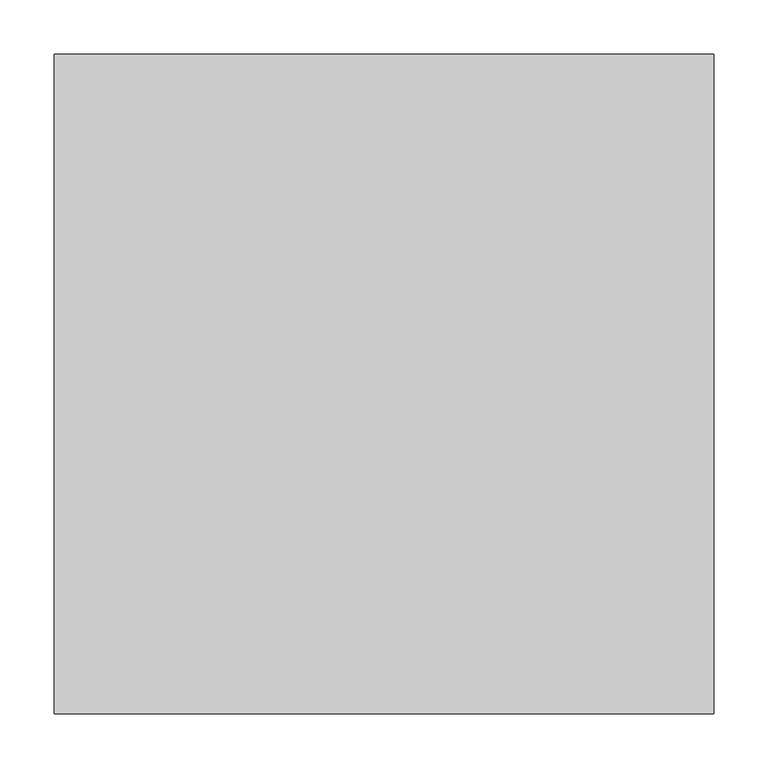
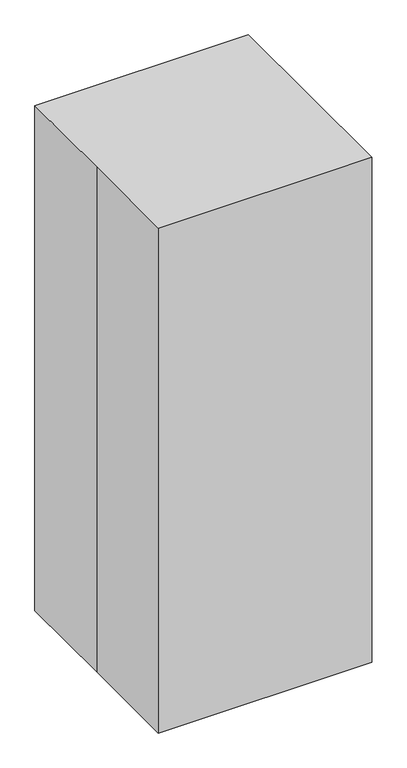
"""IFC4 building model written with IfcOpenShell, lengths in millimetres: proxy geometry, M4116 - Monitor, Vital Signs, On Mobile Stand : M4116 - Monitor, Vital Signs, On Mobile Stand."""

import ifcopenshell
import ifcopenshell.guid

model = None  # the IFC model being written
_history = None  # IfcOwnerHistory: only IFC2X3 demands one
_inside = {}  # id of a spatial element -> (the spatial element, [elements in it])
_under = {}  # id of a project, library or spatial element -> (it, [spatial elements below it])
_declared = {}  # id of a project -> (the project, [libraries it declares])
_typed = {}  # id of a type object -> (the type object, [elements of that type])
_made_of = {}  # id of a material, layer set ... -> (it, [elements and type objects made of it])


def new_model(schema):
    """Start an empty IFC model of exactly this schema.

    Asked for "IFC4X3", IfcOpenShell would pick the latest addendum, in which some entities
    have other attributes; the version numbers below select the first issue.
    IFC2X3 requires an IfcOwnerHistory on every rooted entity: one is made here for all.
    """
    global model, _history
    if schema == "IFC4X3":
        model = ifcopenshell.file(schema_version=(4, 3, 0, 0))
    else:
        model = ifcopenshell.file(schema=schema)
    _inside.clear()
    _under.clear()
    _declared.clear()
    _typed.clear()
    _made_of.clear()
    _history = None
    if model.schema == "IFC2X3":
        org = make("IfcOrganization", Name="unknown")
        user = make(
            "IfcPersonAndOrganization",
            ThePerson=make("IfcPerson", FamilyName="unknown"),
            TheOrganization=org,
        )
        app = make(
            "IfcApplication",
            ApplicationDeveloper=org,
            Version="unknown",
            ApplicationFullName="unknown",
            ApplicationIdentifier="unknown",
        )
        _history = make(
            "IfcOwnerHistory",
            OwningUser=user,
            OwningApplication=app,
            ChangeAction="ADDED",
            CreationDate=0,
        )
    return model


def make(cls, **values):
    """One entity of the class cls with the attributes given. An attribute that is None is left unset."""
    return model.create_entity(
        cls, **{name: value for name, value in values.items() if value is not None}
    )


def rooted(cls, **values):
    """An entity with a GlobalId (a new one), such as an element, a storey or a relation."""
    return make(cls, GlobalId=ifcopenshell.guid.new(), OwnerHistory=_history, **values)


def si_unit(unit_type, name, prefix=None):
    """IfcSIUnit, for example si_unit("LENGTHUNIT", "METRE", prefix="MILLI")."""
    return make("IfcSIUnit", UnitType=unit_type, Prefix=prefix, Name=name)


def assignment(units):
    """IfcUnitAssignment: the units of a project."""
    return None if units is None else make("IfcUnitAssignment", Units=units)


def point(xyz):
    """IfcCartesianPoint."""
    return None if xyz is None else make("IfcCartesianPoint", Coordinates=xyz)


def direction(xyz):
    """IfcDirection."""
    return None if xyz is None else make("IfcDirection", DirectionRatios=xyz)


def frame(location, z_axis=None, x_axis=None):
    """IfcAxis2Placement3D, a coordinate frame: its origin and axes. An axis left out is left unset."""
    return make(
        "IfcAxis2Placement3D",
        Location=point(location),
        Axis=direction(z_axis),
        RefDirection=direction(x_axis),
    )


def frame_2d(location, x_axis=None):
    """IfcAxis2Placement2D, a coordinate frame in the plane: its origin and x axis."""
    return make(
        "IfcAxis2Placement2D", Location=point(location), RefDirection=direction(x_axis)
    )


def origin():
    """The frame at (0, 0, 0) with its axes left unset."""
    return frame((0.0, 0.0, 0.0))


def origin_with_axes():
    """The frame at (0, 0, 0) with the z axis (0, 0, 1) and the x axis (1, 0, 0) written out."""
    return frame((0.0, 0.0, 0.0), z_axis=(0.0, 0.0, 1.0), x_axis=(1.0, 0.0, 0.0))


def origin_2d():
    """The frame at (0, 0) in the plane with its x axis left unset."""
    return frame_2d((0.0, 0.0))


def place(relative_to, where):
    """IfcLocalPlacement: puts the frame where relative to a parent placement (None: the world)."""
    return make(
        "IfcLocalPlacement", PlacementRelTo=relative_to, RelativePlacement=where
    )


def context(
    kind, dimensions, precision=None, world=None, true_north=None, identifier=None
):
    """IfcGeometricRepresentationContext, for example the 3D "Model" context."""
    return make(
        "IfcGeometricRepresentationContext",
        ContextIdentifier=identifier,
        ContextType=kind,
        CoordinateSpaceDimension=dimensions,
        Precision=precision,
        WorldCoordinateSystem=world,
        TrueNorth=true_north,
    )


def project(units=None, contexts=None):
    """IfcProject with its units and contexts."""
    return rooted(
        "IfcProject",
        Name="project",
        RepresentationContexts=contexts,
        UnitsInContext=assignment(units),
    )


def spatial(cls, under=None, at=None, **own):
    """A site, building, storey or space (cls), placed at a placement, below another one or the project."""
    s = rooted(cls, ObjectPlacement=at, **own)
    if under is not None:
        _under.setdefault(under.id(), (under, []))[1].append(s)
    return s


def polyline(points):
    """IfcPolyline through the points."""
    return make("IfcPolyline", Points=[point(p) for p in points])


def circle_curve(where, radius):
    """IfcCircle in the frame where."""
    return make("IfcCircle", Position=where, Radius=radius)


def ellipse_curve(where, semi_axis1, semi_axis2):
    """IfcEllipse in the frame where."""
    return make(
        "IfcEllipse", Position=where, SemiAxis1=semi_axis1, SemiAxis2=semi_axis2
    )


def trimmed(basis, trim1, trim2, sense, master):
    """IfcTrimmedCurve: the piece of a basis curve between two trims."""
    return make(
        "IfcTrimmedCurve",
        BasisCurve=basis,
        Trim1=trim1,
        Trim2=trim2,
        SenseAgreement=sense,
        MasterRepresentation=master,
    )


def segment(curve, same_sense, transition):
    """IfcCompositeCurveSegment."""
    return make(
        "IfcCompositeCurveSegment",
        Transition=transition,
        SameSense=same_sense,
        ParentCurve=curve,
    )


def composite_curve(segments, self_intersect=None):
    """IfcCompositeCurve: segments joined end to end."""
    return make("IfcCompositeCurve", Segments=segments, SelfIntersect=self_intersect)


def outline(outer, holes=None, kind="AREA"):
    """IfcArbitraryClosedProfileDef: a profile drawn as a closed curve; with holes, ...WithVoids."""
    if holes is None:
        return make("IfcArbitraryClosedProfileDef", ProfileType=kind, OuterCurve=outer)
    return make(
        "IfcArbitraryProfileDefWithVoids",
        ProfileType=kind,
        OuterCurve=outer,
        InnerCurves=holes,
    )


def extrude(swept, where, along, depth):
    """IfcExtrudedAreaSolid: the profile swept, set in the frame where, extruded along a direction by depth."""
    return make(
        "IfcExtrudedAreaSolid",
        SweptArea=swept,
        Position=where,
        ExtrudedDirection=direction(along),
        Depth=depth,
    )


def shape(context_of_items, identifier, shape_type, items):
    """IfcShapeRepresentation: the items that make up one representation, for example the "Body"."""
    return make(
        "IfcShapeRepresentation",
        ContextOfItems=context_of_items,
        RepresentationIdentifier=identifier,
        RepresentationType=shape_type,
        Items=items,
    )


def source(mapping_origin, context_of_items, identifier, shape_type, items):
    """IfcRepresentationMap: a shape defined once, which mapped items show again and again."""
    return make(
        "IfcRepresentationMap",
        MappingOrigin=mapping_origin,
        MappedRepresentation=shape(context_of_items, identifier, shape_type, items),
    )


def transform(
    local_origin,
    x_axis=None,
    y_axis=None,
    z_axis=None,
    scale=None,
    scale2=None,
    scale3=None,
    uniform=True,
):
    """IfcCartesianTransformationOperator3D, or its non-uniform kind. x_axis, y_axis, z_axis: its Axis1, 2, 3."""
    if uniform:
        return make(
            "IfcCartesianTransformationOperator3D",
            Axis1=direction(x_axis),
            Axis2=direction(y_axis),
            LocalOrigin=point(local_origin),
            Scale=scale,
            Axis3=direction(z_axis),
        )
    return make(
        "IfcCartesianTransformationOperator3DnonUniform",
        Axis1=direction(x_axis),
        Axis2=direction(y_axis),
        LocalOrigin=point(local_origin),
        Scale=scale,
        Axis3=direction(z_axis),
        Scale2=scale2,
        Scale3=scale3,
    )


def mapped(mapping_source, mapping_target):
    """IfcMappedItem: shows the shape of a source again, moved by a transform."""
    return make(
        "IfcMappedItem", MappingSource=mapping_source, MappingTarget=mapping_target
    )


def made_of(thing, what):
    """Note that an element or type object is made of a material, layer set ...; save() writes the relation."""
    if what is not None:
        _made_of.setdefault(what.id(), (what, []))[1].append(thing)
    return thing


def element(
    cls,
    number,
    at=None,
    inside=None,
    cuts=None,
    type_object=None,
    material=None,
    context=None,
    identifier="Body",
    shape_type=None,
    held_by="IfcProductDefinitionShape",
    body=None,
    shapes=None,
    **own,
):
    """One element of the class cls, such as IfcWall. Its Tag is "e" and its number.

    at: its placement. inside: the storey or other place that contains it. cuts: it is an
    opening in that element (IfcRelVoidsElement). A single representation is given by context,
    identifier, shape_type and body (its items); several are given by shapes. held_by: the class
    of the entity that holds the representations. save() writes the other relations.
    """
    e = rooted(cls, Tag="e%d" % number, ObjectPlacement=at, **own)
    if body is not None:
        shapes = [shape(context, identifier, shape_type, body)]
    if shapes is not None:
        e.Representation = make(held_by, Representations=shapes)
    if inside is not None:
        _inside.setdefault(inside.id(), (inside, []))[1].append(e)
    if cuts is not None:
        rooted(
            "IfcRelVoidsElement", RelatingBuildingElement=cuts, RelatedOpeningElement=e
        )
    if type_object is not None:
        _typed.setdefault(type_object.id(), (type_object, []))[1].append(e)
    return made_of(e, material)


def aggregate(whole, parts):
    """IfcRelAggregates: a whole, such as a stair, and the parts it consists of."""
    return rooted("IfcRelAggregates", RelatingObject=whole, RelatedObjects=parts)


def save(model, path):
    """Write the relations noted so far, then the file.

    IfcRelAggregates (storeys below a building ...), IfcRelContainedInSpatialStructure (elements
    in a storey), IfcRelDefinesByType, IfcRelAssociatesMaterial and IfcRelDeclares: one each for
    every whole, place, type object, material and project.
    """
    for whole, parts in _under.values():
        aggregate(whole, parts)
    for where, things in _inside.values():
        rooted(
            "IfcRelContainedInSpatialStructure",
            RelatedElements=things,
            RelatingStructure=where,
        )
    for kind, things in _typed.values():
        rooted("IfcRelDefinesByType", RelatedObjects=things, RelatingType=kind)
    for what, things in _made_of.values():
        rooted("IfcRelAssociatesMaterial", RelatedObjects=things, RelatingMaterial=what)
    for by, libraries in _declared.values():
        rooted("IfcRelDeclares", RelatingContext=by, RelatedDefinitions=libraries)
    model.write(path)


def plane_surface(at):
    """IfcPlane: the flat surface through the origin of the frame at, square to its z axis."""
    return make("IfcPlane", Position=at)


def cylinder_surface(at, radius):
    """IfcCylindricalSurface: all points at the distance radius from the z axis of the frame at."""
    return make("IfcCylindricalSurface", Position=at, Radius=radius)


def advanced_brep(points, edges, surfaces, faces):
    """IfcAdvancedBrep: a solid bounded by faces that lie on surfaces and meet in shared edges.

    An edge is (start, end): straight between two places in points (the first is 0);
    or (start, end, curve); or (start, end, curve, False) where it runs against its curve.
    A face is (place in surfaces, loops), or (place, loops, False) where it looks against
    its surface's normal. A loop lists edges by number (the first is 1), with a minus sign
    where the edge is run from its end to its start. The first loop is the outer one.
    """
    corners = [point(p) for p in points]
    vertices = [make("IfcVertexPoint", VertexGeometry=c) for c in corners]
    made = []
    for start, end, *more in edges:
        made.append(
            make(
                "IfcEdgeCurve",
                EdgeStart=vertices[start],
                EdgeEnd=vertices[end],
                EdgeGeometry=more[0] if more else make("IfcPolyline", Points=[corners[start], corners[end]]),
                SameSense=more[1] if len(more) > 1 else True,
            )
        )
    hull = []
    for where, loops, *sense in faces:
        bounds = []
        for j, loop in enumerate(loops):
            ring = [make("IfcOrientedEdge", EdgeElement=made[abs(k) - 1], Orientation=k > 0) for k in loop]
            bounds.append(
                make(
                    "IfcFaceOuterBound" if j == 0 else "IfcFaceBound",
                    Bound=make("IfcEdgeLoop", EdgeList=ring),
                    Orientation=True,
                )
            )
        hull.append(make("IfcAdvancedFace", Bounds=bounds, FaceSurface=surfaces[where], SameSense=sense[0] if sense else True))
    return make("IfcAdvancedBrep", Outer=make("IfcClosedShell", CfsFaces=hull))


def specialty_equipment_00fe3c99(model_context):
    return source(origin(), model_context, "Body", "SolidModel", [
        advanced_brep(
        [(-98.425, -113.0619845, 1003.3), (-79.375, -113.0619845, 1003.3), (-98.425, -173.3869845, 1003.3), (-79.375, -154.3369845, 1003.3), (98.425, -173.3869845, 1003.3), (79.375, -154.3369845, 1003.3), (98.425, -113.0619845, 1003.3), (79.375, -113.0619845, 1003.3)],
        [
            (0, 1, circle_curve(frame((-88.9, -113.0619845, 1003.3), z_axis=(0.0, 1.0, 0.0), x_axis=(1.0, 0.0, 0.0)), 9.525)),
            (1, 0, circle_curve(frame((-88.9, -113.0619845, 1003.3), z_axis=(0.0, 1.0, 0.0), x_axis=(1.0, 0.0, 0.0)), 9.525)),
            (0, 2),
            (2, 3, ellipse_curve(frame((-88.9, -163.8619845, 1003.3), z_axis=(-0.7071067811865462, 0.7071067811865487, 0.0), x_axis=(0.7071067811865486, 0.7071067811865464, 0.0)), 13.4703842, 9.525)),
            (3, 1),
            (3, 2, ellipse_curve(frame((-88.9, -163.8619845, 1003.3), z_axis=(-0.7071067811865462, 0.7071067811865487, 0.0), x_axis=(0.7071067811865486, 0.7071067811865464, 0.0)), 13.4703842, 9.525)),
            (2, 4),
            (4, 5, ellipse_curve(frame((88.9, -163.8619845, 1003.3), z_axis=(-0.7071067811865487, -0.7071067811865462, 0.0), x_axis=(-0.7071067811865464, 0.7071067811865487, 0.0)), 13.4703842, 9.525)),
            (5, 3),
            (5, 4, ellipse_curve(frame((88.9, -163.8619845, 1003.3), z_axis=(-0.7071067811865487, -0.7071067811865462, 0.0), x_axis=(-0.7071067811865464, 0.7071067811865487, 0.0)), 13.4703842, 9.525)),
            (6, 7, circle_curve(frame((88.9, -113.0619845, 1003.3), z_axis=(0.0, 1.0, 0.0), x_axis=(-1.0, 0.0, 0.0)), 9.525)),
            (7, 6, circle_curve(frame((88.9, -113.0619845, 1003.3), z_axis=(0.0, 1.0, 0.0), x_axis=(-1.0, 0.0, 0.0)), 9.525)),
            (4, 6),
            (7, 5),
        ],
        [
            plane_surface(frame((-88.9, -113.0619845, 1003.3), z_axis=(0.0, 1.0, 0.0), x_axis=(0.0, 0.0, 1.0))),
            cylinder_surface(frame((-88.9, -113.0619845, 1003.3), z_axis=(0.0, 1.0, 0.0), x_axis=(1.0, 0.0, 0.0)), 9.525),
            cylinder_surface(frame((-88.9, -163.8619845, 1003.3), z_axis=(-1.0, 0.0, 0.0), x_axis=(0.0, 1.0, 0.0)), 9.525),
            plane_surface(frame((88.9, -113.0619845, 1003.3), z_axis=(0.0, 1.0, 0.0), x_axis=(0.0, 0.0, 1.0))),
            cylinder_surface(frame((88.9, -163.8619845, 1003.3), z_axis=(0.0, -1.0, 0.0), x_axis=(-1.0, 0.0, 0.0)), 9.525),
        ],
        [
            (0, [[1, 2]]),
            (1, [[-1, 3, 4, 5]]),
            (1, [[-2, -5, 6, -3]]),
            (2, [[-4, 7, 8, 9]]),
            (2, [[-6, -9, 10, -7]]),
            (3, [[11, 12]]),
            (4, [[-8, 13, -12, 14]]),
            (4, [[-10, -14, -11, -13]]),
        ],
    ),
        extrude(outline(polyline([(101.6, 965.2), (-113.0619845, 965.2), (-113.0619845, 1036.8125795), (-57.3005542, 1219.2), (101.6, 1219.2), (101.6, 965.2)])), frame((-127.0, 0.0, 0.0), z_axis=(1.0, 0.0, 0.0), x_axis=(0.0, 1.0, 0.0)), (0.0, 0.0, 1.0), 254.0),
        extrude(outline(composite_curve([segment(trimmed(circle_curve(frame_2d((25.4, -203.0677083)), 25.4), [point((25.4, -228.4677083))], [point((25.4, -177.6677083))], False, "CARTESIAN"), True, "CONTINUOUS"), segment(trimmed(circle_curve(frame_2d((25.4, -203.0677083)), 25.4), [point((25.4, -177.6677083))], [point((25.4, -228.4677083))], False, "CARTESIAN"), True, "CONTINUOUS")], self_intersect=False)), frame((0.0, 9.525, 0.0), z_axis=(0.0, 1.0, 0.0), x_axis=(0.0, 0.0, 1.0)), (0.0, 0.0, 1.0), 9.525),
        extrude(outline(composite_curve([segment(trimmed(circle_curve(frame_2d((25.4, -203.0677083)), 25.4), [point((25.4, -177.6677083))], [point((25.4, -228.4677083))], False, "CARTESIAN"), True, "CONTINUOUS"), segment(trimmed(circle_curve(frame_2d((25.4, -203.0677083)), 25.4), [point((25.4, -228.4677083))], [point((25.4, -177.6677083))], False, "CARTESIAN"), True, "CONTINUOUS")], self_intersect=False)), frame((0.0, -19.05, 0.0), z_axis=(0.0, 1.0, 0.0), x_axis=(0.0, 0.0, 1.0)), (0.0, 0.0, 1.0), 9.525),
        extrude(outline(composite_curve([segment(trimmed(circle_curve(frame_2d((203.0677083, 25.4)), 25.4), [point((228.4677083, 25.4))], [point((177.6677083, 25.4))], False, "CARTESIAN"), True, "CONTINUOUS"), segment(trimmed(circle_curve(frame_2d((203.0677083, 25.4)), 25.4), [point((177.6677083, 25.4))], [point((228.4677083, 25.4))], False, "CARTESIAN"), True, "CONTINUOUS")], self_intersect=False)), frame((9.525, 0.0, 0.0), z_axis=(1.0, 0.0, 0.0), x_axis=(0.0, 1.0, 0.0)), (0.0, 0.0, 1.0), 9.525),
        extrude(outline(composite_curve([segment(trimmed(circle_curve(frame_2d((203.0677083, 25.4)), 25.4), [point((177.6677083, 25.4))], [point((228.4677083, 25.4))], False, "CARTESIAN"), True, "CONTINUOUS"), segment(trimmed(circle_curve(frame_2d((203.0677083, 25.4)), 25.4), [point((228.4677083, 25.4))], [point((177.6677083, 25.4))], False, "CARTESIAN"), True, "CONTINUOUS")], self_intersect=False)), frame((-19.05, 0.0, 0.0), z_axis=(1.0, 0.0, 0.0), x_axis=(0.0, 1.0, 0.0)), (0.0, 0.0, 1.0), 9.525),
        extrude(outline(composite_curve([segment(trimmed(circle_curve(frame_2d((25.4, 203.2661458)), 25.4), [point((25.4, 177.8661458))], [point((25.4, 228.6661458))], False, "CARTESIAN"), True, "CONTINUOUS"), segment(trimmed(circle_curve(frame_2d((25.4, 203.2661458)), 25.4), [point((25.4, 228.6661458))], [point((25.4, 177.8661458))], False, "CARTESIAN"), True, "CONTINUOUS")], self_intersect=False)), frame((0.0, -19.05, 0.0), z_axis=(0.0, 1.0, 0.0), x_axis=(0.0, 0.0, 1.0)), (0.0, 0.0, 1.0), 9.525),
        extrude(outline(composite_curve([segment(trimmed(circle_curve(frame_2d((25.4, 203.2661458)), 25.4), [point((25.4, 177.8661458))], [point((25.4, 228.6661458))], False, "CARTESIAN"), True, "CONTINUOUS"), segment(trimmed(circle_curve(frame_2d((25.4, 203.2661458)), 25.4), [point((25.4, 228.6661458))], [point((25.4, 177.8661458))], False, "CARTESIAN"), True, "CONTINUOUS")], self_intersect=False)), frame((0.0, 9.525, 0.0), z_axis=(0.0, 1.0, 0.0), x_axis=(0.0, 0.0, 1.0)), (0.0, 0.0, 1.0), 9.525),
        extrude(outline(composite_curve([segment(trimmed(circle_curve(frame_2d((0.0, 211.534375)), 8.4666667), [point((-8.4666667, 211.534375))], [point((8.4666667, 211.534375))], False, "CARTESIAN"), True, "CONTINUOUS"), segment(trimmed(circle_curve(frame_2d((0.0, 211.534375)), 8.4666667), [point((8.4666667, 211.534375))], [point((-8.4666667, 211.534375))], False, "CARTESIAN"), True, "CONTINUOUS")], self_intersect=False)), frame((0.0, 0.0, 25.4), z_axis=(0.0, 0.0, 1.0), x_axis=(1.0, 0.0, 0.0)), (0.0, 0.0, 1.0), 25.4),
        extrude(outline(composite_curve([segment(trimmed(circle_curve(frame_2d((203.0677083, 25.4)), 16.9333333), [point((186.134375, 25.4))], [point((220.0010417, 25.4))], False, "CARTESIAN"), True, "CONTINUOUS"), segment(trimmed(circle_curve(frame_2d((203.0677083, 25.4)), 16.9333333), [point((220.0010417, 25.4))], [point((186.134375, 25.4))], False, "CARTESIAN"), True, "CONTINUOUS")], self_intersect=False)), frame((-9.525, 0.0, 0.0), z_axis=(1.0, 0.0, 0.0), x_axis=(0.0, 1.0, 0.0)), (0.0, 0.0, 1.0), 19.05),
        extrude(outline(composite_curve([segment(trimmed(circle_curve(frame_2d((211.7328125, 0.0)), 8.4666667), [point((211.7328125, 8.4666667))], [point((211.7328125, -8.4666667))], False, "CARTESIAN"), True, "CONTINUOUS"), segment(trimmed(circle_curve(frame_2d((211.7328125, 0.0)), 8.4666667), [point((211.7328125, -8.4666667))], [point((211.7328125, 8.4666667))], False, "CARTESIAN"), True, "CONTINUOUS")], self_intersect=False)), frame((0.0, 0.0, 25.4), z_axis=(0.0, 0.0, 1.0), x_axis=(1.0, 0.0, 0.0)), (0.0, 0.0, 1.0), 25.4),
        extrude(outline(composite_curve([segment(trimmed(circle_curve(frame_2d((25.4, 203.2661458)), 16.9333333), [point((25.4, 186.3328125))], [point((25.4, 220.1994792))], False, "CARTESIAN"), True, "CONTINUOUS"), segment(trimmed(circle_curve(frame_2d((25.4, 203.2661458)), 16.9333333), [point((25.4, 220.1994792))], [point((25.4, 186.3328125))], False, "CARTESIAN"), True, "CONTINUOUS")], self_intersect=False)), frame((0.0, -9.525, 0.0), z_axis=(0.0, 1.0, 0.0), x_axis=(0.0, 0.0, 1.0)), (0.0, 0.0, 1.0), 19.05),
        extrude(outline(composite_curve([segment(trimmed(circle_curve(frame_2d((-211.534375, 0.0)), 8.4666667), [point((-211.534375, -8.4666667))], [point((-211.534375, 8.4666667))], False, "CARTESIAN"), True, "CONTINUOUS"), segment(trimmed(circle_curve(frame_2d((-211.534375, 0.0)), 8.4666667), [point((-211.534375, 8.4666667))], [point((-211.534375, -8.4666667))], False, "CARTESIAN"), True, "CONTINUOUS")], self_intersect=False)), frame((0.0, 0.0, 25.4), z_axis=(0.0, 0.0, 1.0), x_axis=(1.0, 0.0, 0.0)), (0.0, 0.0, 1.0), 25.4),
        extrude(outline(composite_curve([segment(trimmed(circle_curve(frame_2d((25.4, -203.0677083)), 16.9333333), [point((25.4, -186.134375))], [point((25.4, -220.0010417))], False, "CARTESIAN"), True, "CONTINUOUS"), segment(trimmed(circle_curve(frame_2d((25.4, -203.0677083)), 16.9333333), [point((25.4, -220.0010417))], [point((25.4, -186.134375))], False, "CARTESIAN"), True, "CONTINUOUS")], self_intersect=False)), frame((0.0, -9.525, 0.0), z_axis=(0.0, 1.0, 0.0), x_axis=(0.0, 0.0, 1.0)), (0.0, 0.0, 1.0), 19.05),
        extrude(outline(composite_curve([segment(trimmed(circle_curve(frame_2d((-203.2165365, 25.4)), 25.4), [point((-177.8165365, 25.4))], [point((-228.6165365, 25.4))], False, "CARTESIAN"), True, "CONTINUOUS"), segment(trimmed(circle_curve(frame_2d((-203.2165365, 25.4)), 25.4), [point((-228.6165365, 25.4))], [point((-177.8165365, 25.4))], False, "CARTESIAN"), True, "CONTINUOUS")], self_intersect=False)), frame((-19.05, 0.0, 0.0), z_axis=(1.0, 0.0, 0.0), x_axis=(0.0, 1.0, 0.0)), (0.0, 0.0, 1.0), 9.525),
        extrude(outline(composite_curve([segment(trimmed(circle_curve(frame_2d((-203.2165365, 25.4)), 25.4), [point((-177.8165365, 25.4))], [point((-228.6165365, 25.4))], False, "CARTESIAN"), True, "CONTINUOUS"), segment(trimmed(circle_curve(frame_2d((-203.2165365, 25.4)), 25.4), [point((-228.6165365, 25.4))], [point((-177.8165365, 25.4))], False, "CARTESIAN"), True, "CONTINUOUS")], self_intersect=False)), frame((9.525, 0.0, 0.0), z_axis=(1.0, 0.0, 0.0), x_axis=(0.0, 1.0, 0.0)), (0.0, 0.0, 1.0), 9.525),
        extrude(outline(composite_curve([segment(trimmed(circle_curve(frame_2d((0.0, -211.6832031)), 8.4666667), [point((8.4666667, -211.6832031))], [point((-8.4666667, -211.6832031))], False, "CARTESIAN"), True, "CONTINUOUS"), segment(trimmed(circle_curve(frame_2d((0.0, -211.6832031)), 8.4666667), [point((-8.4666667, -211.6832031))], [point((8.4666667, -211.6832031))], False, "CARTESIAN"), True, "CONTINUOUS")], self_intersect=False)), frame((0.0, 0.0, 25.4), z_axis=(0.0, 0.0, 1.0), x_axis=(1.0, 0.0, 0.0)), (0.0, 0.0, 1.0), 25.4),
        extrude(outline(composite_curve([segment(trimmed(circle_curve(frame_2d((-203.2165365, 25.4)), 16.9333333), [point((-186.2832031, 25.4))], [point((-220.1498698, 25.4))], False, "CARTESIAN"), True, "CONTINUOUS"), segment(trimmed(circle_curve(frame_2d((-203.2165365, 25.4)), 16.9333333), [point((-220.1498698, 25.4))], [point((-186.2832031, 25.4))], False, "CARTESIAN"), True, "CONTINUOUS")], self_intersect=False)), frame((-9.525, 0.0, 0.0), z_axis=(1.0, 0.0, 0.0), x_axis=(0.0, 1.0, 0.0)), (0.0, 0.0, 1.0), 19.05),
        extrude(outline(polyline([(-228.6, 63.5), (-192.6166667, 63.5), (-44.45, 25.4), (44.45, 25.4), (192.6166667, 63.5), (228.6, 63.5), (228.6, 50.8), (193.8216772, 50.8), (45.6550105, 12.7), (-45.6550105, 12.7), (-193.8216772, 50.8), (-228.6, 50.8), (-228.6, 63.5)])), frame((-19.05, 0.0, 0.0), z_axis=(1.0, 0.0, 0.0), x_axis=(0.0, 1.0, 0.0)), (0.0, 0.0, 1.0), 38.1),
        extrude(outline(composite_curve([segment(trimmed(circle_curve(origin_2d(), 12.7), [point((-12.7, 0.0))], [point((12.7, 0.0))], False, "CARTESIAN"), True, "CONTINUOUS"), segment(trimmed(circle_curve(origin_2d(), 12.7), [point((12.7, 0.0))], [point((-12.7, 0.0))], False, "CARTESIAN"), True, "CONTINUOUS")], self_intersect=False)), frame((0.0, 0.0, 12.7), z_axis=(0.0, 0.0, 1.0), x_axis=(1.0, 0.0, 0.0)), (0.0, 0.0, 1.0), 952.5),
        extrude(outline(polyline([(63.5, -228.6), (50.8, -228.6), (50.8, -193.8216772), (12.7, -45.6550105), (12.7, 45.6550105), (50.8, 193.8216772), (50.8, 228.6), (63.5, 228.6), (63.5, 192.6166667), (25.4, 44.45), (25.4, -44.45), (63.5, -192.6166667), (63.5, -228.6)])), frame((0.0, -19.05, 0.0), z_axis=(0.0, 1.0, 0.0), x_axis=(0.0, 0.0, 1.0)), (0.0, 0.0, 1.0), 38.1),
        extrude(outline(polyline([(-304.8, 304.8), (304.8, 304.8), (304.8, -304.8), (-304.8, -304.8), (-304.8, 0.0), (-304.8, 304.8)])), origin_with_axes(), (0.0, 0.0, 1.0), 1524.0),
    ])


if __name__ == "__main__":
    model = new_model("IFC4")
    model_context = context("Model", 3, world=origin())
    ifc_project = project(units=[si_unit("LENGTHUNIT", "METRE", prefix="MILLI")], contexts=[model_context])
    site = spatial("IfcSite", under=ifc_project)
    building = spatial("IfcBuilding", under=site)
    placement = place(None, origin())
    specialty_equipment_shape = specialty_equipment_00fe3c99(model_context)
    element("IfcBuildingElementProxy", 1, Name="M4116 - Monitor, Vital Signs, On Mobile Stand : M4116 - Monitor, Vital Signs, On Mobile Stand", ObjectType="M4116 - Monitor, Vital Signs, On Mobile Stand : M4116 - Monitor, Vital Signs, On Mobile Stand", at=placement, inside=building, context=model_context, shape_type="MappedRepresentation", body=[
        mapped(specialty_equipment_shape, transform((0.0, 0.0, 0.0), x_axis=(1.0, 0.0, 0.0), y_axis=(0.0, 1.0, 0.0), z_axis=(0.0, 0.0, 1.0))),
    ])
    save(model, "model.ifc")

# Revit data of these elements
# Project information
#   Sheets - Total = "7"
#   Project Issue Date = "Issue Date"
#   Project Status = "Project Status"
#   Client Name = "Owner"
#   Project Address = "Enter address here"
#   Project Name = "Project Name"
#   Project Number = "Project Number"
#   Publication Date = "30-Jan-15"
# Type "M4116 - Monitor, Vital Signs, On Mobile Stand : M4116 - Monitor, Vital Signs, On Mobile Stand"
#   Watts2 = "0"
#   Watts1 = "240"
#   Unit_Issue = "EA"
#   UTIL_6_Misc = "-"
#   UTIL_5_NonMedGas = "-"
#   UTIL_4_MiscGas = "-"
#   UTIL_3_MedGas = "-"
#   UTIL_2_Elec = "A"
#   UTIL_1_WaterDrain = "-"
#   Nomenclature = "Monitor, Vital Signs"
#   NSN = "6515"
#   Location [instance default] = ""
#   JSN = "M4116"
#   Fund_Source_VA = "-"
#   Fund_Source_Navy = "-"
#   Fund_Source_Army = "-"
#   Fund_Source_AF = "-"
#   ELEC_Volts2 = "0"
#   ELEC_Volts1 = "120"
#   ELEC_Phase2 = "0"
#   ELEC_Phase1 = "1"
#   ELEC_HertzSwitch = "60"
#   ELEC_HertzDependent = "0"
#   ELEC_Hertz = "0"
#   ELEC_Amps2 = "0"
#   ELEC_Amps1 = "2"
#   DetailDescription = "Electronic sphygmomanometer. LCD displays non-invasive blood pressure, pulse rate and temperature. Used in hospitals and clinics. Includes an optional mobile stand."
#   CAT_VA = "C"
#   CAT_Navy = "C"
#   CAT_IHS = "-"
#   CAT_Army = "C"
#   CAT_AF = "C"
#   BTUperhour = "0"
#   Weight_IP = 40
#   DIM_Width_IP = 2' - 0"
#   DIM_Height_IP = 5' - 0"
#   DIM_Depth_IP = 2' - 0"
#   finish [instance default] = none
# Element 1 (IfcBuildingElementProxy, "M4116 - Monitor, Vital Signs, On Mobile Stand : M4116 - Monitor, Vital Signs, On Mobile Stand")
#   Location = "LDAT2"
#   Materials on its faces: "EquipSpace"
# Materials
#   "EquipSpace": class "Unassigned", colour RGB 221 217 195, transparency 0.5
